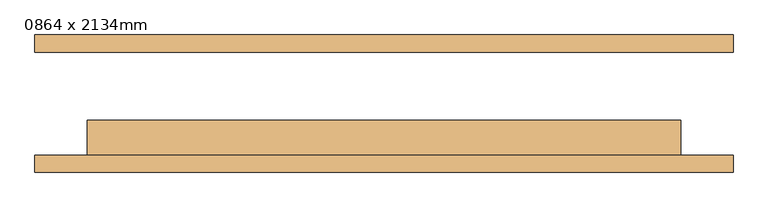
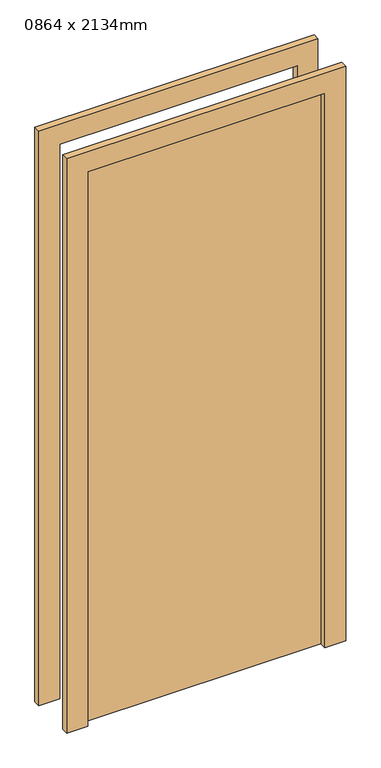
"""IFC4 building model written with IfcOpenShell, lengths in millimetres: door geometry, M_Folha única : 0864 x 2134mm."""

import ifcopenshell
import ifcopenshell.guid

model = None  # the IFC model being written
_history = None  # IfcOwnerHistory: only IFC2X3 demands one
_inside = {}  # id of a spatial element -> (the spatial element, [elements in it])
_under = {}  # id of a project, library or spatial element -> (it, [spatial elements below it])
_declared = {}  # id of a project -> (the project, [libraries it declares])
_typed = {}  # id of a type object -> (the type object, [elements of that type])
_made_of = {}  # id of a material, layer set ... -> (it, [elements and type objects made of it])


def new_model(schema):
    """Start an empty IFC model of exactly this schema.

    Asked for "IFC4X3", IfcOpenShell would pick the latest addendum, in which some entities
    have other attributes; the version numbers below select the first issue.
    IFC2X3 requires an IfcOwnerHistory on every rooted entity: one is made here for all.
    """
    global model, _history
    if schema == "IFC4X3":
        model = ifcopenshell.file(schema_version=(4, 3, 0, 0))
    else:
        model = ifcopenshell.file(schema=schema)
    _inside.clear()
    _under.clear()
    _declared.clear()
    _typed.clear()
    _made_of.clear()
    _history = None
    if model.schema == "IFC2X3":
        org = make("IfcOrganization", Name="unknown")
        user = make(
            "IfcPersonAndOrganization",
            ThePerson=make("IfcPerson", FamilyName="unknown"),
            TheOrganization=org,
        )
        app = make(
            "IfcApplication",
            ApplicationDeveloper=org,
            Version="unknown",
            ApplicationFullName="unknown",
            ApplicationIdentifier="unknown",
        )
        _history = make(
            "IfcOwnerHistory",
            OwningUser=user,
            OwningApplication=app,
            ChangeAction="ADDED",
            CreationDate=0,
        )
    return model


def make(cls, **values):
    """One entity of the class cls with the attributes given. An attribute that is None is left unset."""
    return model.create_entity(
        cls, **{name: value for name, value in values.items() if value is not None}
    )


def rooted(cls, **values):
    """An entity with a GlobalId (a new one), such as an element, a storey or a relation."""
    return make(cls, GlobalId=ifcopenshell.guid.new(), OwnerHistory=_history, **values)


def si_unit(unit_type, name, prefix=None):
    """IfcSIUnit, for example si_unit("LENGTHUNIT", "METRE", prefix="MILLI")."""
    return make("IfcSIUnit", UnitType=unit_type, Prefix=prefix, Name=name)


def assignment(units):
    """IfcUnitAssignment: the units of a project."""
    return None if units is None else make("IfcUnitAssignment", Units=units)


def point(xyz):
    """IfcCartesianPoint."""
    return None if xyz is None else make("IfcCartesianPoint", Coordinates=xyz)


def direction(xyz):
    """IfcDirection."""
    return None if xyz is None else make("IfcDirection", DirectionRatios=xyz)


def frame(location, z_axis=None, x_axis=None):
    """IfcAxis2Placement3D, a coordinate frame: its origin and axes. An axis left out is left unset."""
    return make(
        "IfcAxis2Placement3D",
        Location=point(location),
        Axis=direction(z_axis),
        RefDirection=direction(x_axis),
    )


def origin():
    """The frame at (0, 0, 0) with its axes left unset."""
    return frame((0.0, 0.0, 0.0))


def origin_with_axes():
    """The frame at (0, 0, 0) with the z axis (0, 0, 1) and the x axis (1, 0, 0) written out."""
    return frame((0.0, 0.0, 0.0), z_axis=(0.0, 0.0, 1.0), x_axis=(1.0, 0.0, 0.0))


def place(relative_to, where):
    """IfcLocalPlacement: puts the frame where relative to a parent placement (None: the world)."""
    return make(
        "IfcLocalPlacement", PlacementRelTo=relative_to, RelativePlacement=where
    )


def context(
    kind, dimensions, precision=None, world=None, true_north=None, identifier=None
):
    """IfcGeometricRepresentationContext, for example the 3D "Model" context."""
    return make(
        "IfcGeometricRepresentationContext",
        ContextIdentifier=identifier,
        ContextType=kind,
        CoordinateSpaceDimension=dimensions,
        Precision=precision,
        WorldCoordinateSystem=world,
        TrueNorth=true_north,
    )


def project(units=None, contexts=None):
    """IfcProject with its units and contexts."""
    return rooted(
        "IfcProject",
        Name="project",
        RepresentationContexts=contexts,
        UnitsInContext=assignment(units),
    )


def spatial(cls, under=None, at=None, **own):
    """A site, building, storey or space (cls), placed at a placement, below another one or the project."""
    s = rooted(cls, ObjectPlacement=at, **own)
    if under is not None:
        _under.setdefault(under.id(), (under, []))[1].append(s)
    return s


def polyline(points):
    """IfcPolyline through the points."""
    return make("IfcPolyline", Points=[point(p) for p in points])


def outline(outer, holes=None, kind="AREA"):
    """IfcArbitraryClosedProfileDef: a profile drawn as a closed curve; with holes, ...WithVoids."""
    if holes is None:
        return make("IfcArbitraryClosedProfileDef", ProfileType=kind, OuterCurve=outer)
    return make(
        "IfcArbitraryProfileDefWithVoids",
        ProfileType=kind,
        OuterCurve=outer,
        InnerCurves=holes,
    )


def extrude(swept, where, along, depth):
    """IfcExtrudedAreaSolid: the profile swept, set in the frame where, extruded along a direction by depth."""
    return make(
        "IfcExtrudedAreaSolid",
        SweptArea=swept,
        Position=where,
        ExtrudedDirection=direction(along),
        Depth=depth,
    )


def shape(context_of_items, identifier, shape_type, items):
    """IfcShapeRepresentation: the items that make up one representation, for example the "Body"."""
    return make(
        "IfcShapeRepresentation",
        ContextOfItems=context_of_items,
        RepresentationIdentifier=identifier,
        RepresentationType=shape_type,
        Items=items,
    )


def source(mapping_origin, context_of_items, identifier, shape_type, items):
    """IfcRepresentationMap: a shape defined once, which mapped items show again and again."""
    return make(
        "IfcRepresentationMap",
        MappingOrigin=mapping_origin,
        MappedRepresentation=shape(context_of_items, identifier, shape_type, items),
    )


def transform(
    local_origin,
    x_axis=None,
    y_axis=None,
    z_axis=None,
    scale=None,
    scale2=None,
    scale3=None,
    uniform=True,
):
    """IfcCartesianTransformationOperator3D, or its non-uniform kind. x_axis, y_axis, z_axis: its Axis1, 2, 3."""
    if uniform:
        return make(
            "IfcCartesianTransformationOperator3D",
            Axis1=direction(x_axis),
            Axis2=direction(y_axis),
            LocalOrigin=point(local_origin),
            Scale=scale,
            Axis3=direction(z_axis),
        )
    return make(
        "IfcCartesianTransformationOperator3DnonUniform",
        Axis1=direction(x_axis),
        Axis2=direction(y_axis),
        LocalOrigin=point(local_origin),
        Scale=scale,
        Axis3=direction(z_axis),
        Scale2=scale2,
        Scale3=scale3,
    )


def mapped(mapping_source, mapping_target):
    """IfcMappedItem: shows the shape of a source again, moved by a transform."""
    return make(
        "IfcMappedItem", MappingSource=mapping_source, MappingTarget=mapping_target
    )


def made_of(thing, what):
    """Note that an element or type object is made of a material, layer set ...; save() writes the relation."""
    if what is not None:
        _made_of.setdefault(what.id(), (what, []))[1].append(thing)
    return thing


def element(
    cls,
    number,
    at=None,
    inside=None,
    cuts=None,
    type_object=None,
    material=None,
    context=None,
    identifier="Body",
    shape_type=None,
    held_by="IfcProductDefinitionShape",
    body=None,
    shapes=None,
    **own,
):
    """One element of the class cls, such as IfcWall. Its Tag is "e" and its number.

    at: its placement. inside: the storey or other place that contains it. cuts: it is an
    opening in that element (IfcRelVoidsElement). A single representation is given by context,
    identifier, shape_type and body (its items); several are given by shapes. held_by: the class
    of the entity that holds the representations. save() writes the other relations.
    """
    e = rooted(cls, Tag="e%d" % number, ObjectPlacement=at, **own)
    if body is not None:
        shapes = [shape(context, identifier, shape_type, body)]
    if shapes is not None:
        e.Representation = make(held_by, Representations=shapes)
    if inside is not None:
        _inside.setdefault(inside.id(), (inside, []))[1].append(e)
    if cuts is not None:
        rooted(
            "IfcRelVoidsElement", RelatingBuildingElement=cuts, RelatedOpeningElement=e
        )
    if type_object is not None:
        _typed.setdefault(type_object.id(), (type_object, []))[1].append(e)
    return made_of(e, material)


def aggregate(whole, parts):
    """IfcRelAggregates: a whole, such as a stair, and the parts it consists of."""
    return rooted("IfcRelAggregates", RelatingObject=whole, RelatedObjects=parts)


def save(model, path):
    """Write the relations noted so far, then the file.

    IfcRelAggregates (storeys below a building ...), IfcRelContainedInSpatialStructure (elements
    in a storey), IfcRelDefinesByType, IfcRelAssociatesMaterial and IfcRelDeclares: one each for
    every whole, place, type object, material and project.
    """
    for whole, parts in _under.values():
        aggregate(whole, parts)
    for where, things in _inside.values():
        rooted(
            "IfcRelContainedInSpatialStructure",
            RelatedElements=things,
            RelatingStructure=where,
        )
    for kind, things in _typed.values():
        rooted("IfcRelDefinesByType", RelatedObjects=things, RelatingType=kind)
    for what, things in _made_of.values():
        rooted("IfcRelAssociatesMaterial", RelatedObjects=things, RelatingMaterial=what)
    for by, libraries in _declared.values():
        rooted("IfcRelDeclares", RelatingContext=by, RelatedDefinitions=libraries)
    model.write(path)


def door_0864_x_2134mm_0748c0c9(model_context):
    return source(origin(), model_context, "Body", "SweptSolid", [
        extrude(outline(polyline([(2210.0, -508.0), (0.0, -508.0), (0.0, -432.0), (2134.0, -432.0), (2134.0, 432.0), (0.0, 432.0), (0.0, 508.0), (2210.0, 508.0), (2210.0, -508.0)])), frame((0.0, -100.0, 0.0), z_axis=(0.0, 1.0, 0.0), x_axis=(0.0, 0.0, 1.0)), (0.0, 0.0, 1.0), 25.0),
        extrude(outline(polyline([(2210.0, 508.0), (2210.0, -508.0), (0.0, -508.0), (0.0, -432.0), (2134.0, -432.0), (2134.0, 432.0), (0.0, 432.0), (0.0, 508.0), (2210.0, 508.0)])), frame((0.0, 75.0, 0.0), z_axis=(0.0, 1.0, 0.0), x_axis=(0.0, 0.0, 1.0)), (0.0, 0.0, 1.0), 25.0),
        extrude(outline(polyline([(432.0, -24.0), (432.0, -75.0), (-432.0, -75.0), (-432.0, -24.0), (432.0, -24.0)])), origin_with_axes(), (0.0, 0.0, 1.0), 2134.0),
    ])


if __name__ == "__main__":
    model = new_model("IFC4")
    model_context = context("Model", 3, world=origin())
    ifc_project = project(units=[si_unit("LENGTHUNIT", "METRE", prefix="MILLI")], contexts=[model_context])
    site = spatial("IfcSite", under=ifc_project)
    building = spatial("IfcBuilding", under=site)
    placement = place(None, origin())
    door_0864_x_2134mm_shape = door_0864_x_2134mm_0748c0c9(model_context)
    element("IfcDoor", 1, ObjectType="M_Folha única : 0864 x 2134mm", at=placement, inside=building, context=model_context, shape_type="MappedRepresentation", body=[
        mapped(door_0864_x_2134mm_shape, transform((0.0, 0.0, 0.0), x_axis=(1.0, 0.0, 0.0), y_axis=(0.0, 1.0, 0.0), z_axis=(0.0, 0.0, 1.0))),
    ])
    save(model, "model.ifc")

# Revit data of these elements
# Type "M_Folha única : 0864 x 2134mm"
#   Type Mark = "22"
#   Construction Type Id = "MDOOR"
#   Analytic Construction = "Metal"
#   Thickness = 0.051 m
#   Thermal Resistance (R) = 0.270117 (m²·K)/W
#   Heat Transfer Coefficient (U) = 3.7021 W/(m²·K)
#   Height = 2.134 m
#   Projeção da apara externa = 0.025 m
#   Projeção da apara interna = 0.025 m
#   Largura da apara = 0.076 m
#   Width = 0.864 m
#   Define Thermal Properties by = 1
#   Material da porta = Porta - Painel
#   Material da moldura = Porta - Batente
#   Visual Light Transmittance = 0
#   Solar Heat Gain Coefficient = 0
#   Function = (empty or 0)
#   Wall Closure = (empty or 0)
# Element 1 (IfcDoor, "M_Folha única : 0864 x 2134mm")
#   Materials on its faces: "Porta - Batente", "Porta - Painel"
# Materials
#   "Porta - Painel": class "Madeira", colour RGB 210 159 95, transparency 0, Cost = 0
#   "Porta - Batente": class "Diversos", colour RGB 118 70 51, transparency 0, Cost = 0
